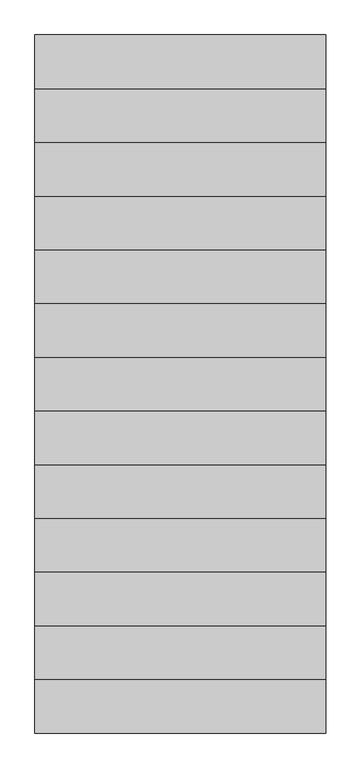
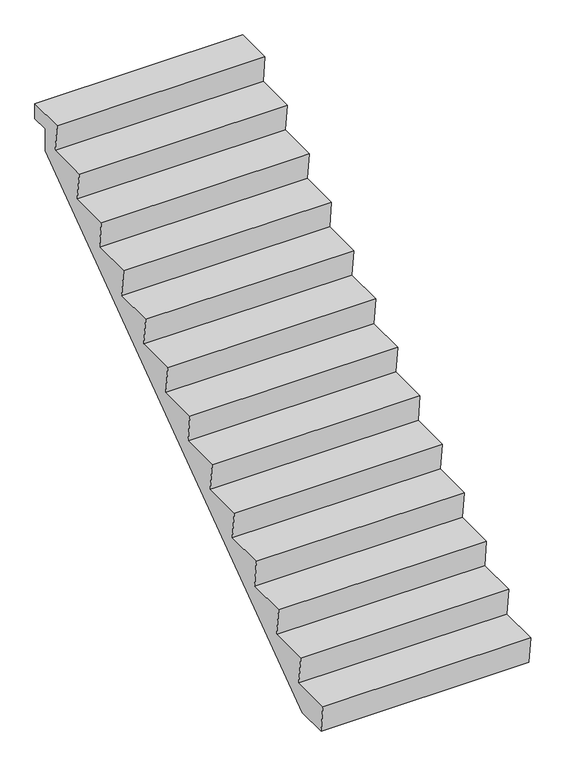
"""IFC4 building model written with IfcOpenShell, lengths in millimetres: stair geometry, NLRS_24_GM_LB_rechte steektrap prefab-AV_gen_rsf : prefab trap_gen__aant=12 b=1200 a=220 o=172.7 zonder bomen."""

from ifc_helpers import new_model, si_unit, frame, origin, place, context, project, spatial, polyline, outline, extrude, source, transform, mapped, element, save


def stair_322cbe82(model_context):
    return source(origin(), model_context, "Body", "SweptSolid", [
        extrude(outline(polyline([(2880.0, 2270.0), (3120.0, 2270.0), (3120.0, 2170.0), (3010.0, 2170.0), (3010.0, 2027.0164203), (223.9686206, 0.0), (20.0, 0.0), (0.0, 174.6153846), (260.0, 174.6153846), (240.0, 349.2307692), (500.0, 349.2307692), (480.0, 523.8461538), (740.0, 523.8461538), (720.0, 698.4615385), (980.0, 698.4615385), (960.0, 873.0769231), (1220.0, 873.0769231), (1200.0, 1047.6923077), (1460.0, 1047.6923077), (1440.0, 1222.3076923), (1700.0, 1222.3076923), (1680.0, 1396.9230769), (1940.0, 1396.9230769), (1920.0, 1571.5384615), (2180.0, 1571.5384615), (2160.0, 1746.1538462), (2420.0, 1746.1538462), (2400.0, 1920.7692308), (2660.0, 1920.7692308), (2640.0, 2095.3846154), (2900.0, 2095.3846154), (2880.0, 2270.0)])), frame((-650.0, 0.0, 0.0), z_axis=(1.0, 0.0, 0.0), x_axis=(0.0, 1.0, 0.0)), (0.0, 0.0, 1.0), 1300.0),
    ])


if __name__ == "__main__":
    model = new_model("IFC4")
    model_context = context("Model", 3, world=origin())
    ifc_project = project(units=[si_unit("LENGTHUNIT", "METRE", prefix="MILLI")], contexts=[model_context])
    site = spatial("IfcSite", under=ifc_project)
    building = spatial("IfcBuilding", under=site)
    placement = place(None, origin())
    stair_shape = stair_322cbe82(model_context)
    element("IfcStair", 1, ObjectType="NLRS_24_GM_LB_rechte steektrap prefab-AV_gen_rsf : prefab trap_gen__aant=12 b=1200 a=220 o=172.7 zonder bomen", at=placement, inside=building, context=model_context, shape_type="MappedRepresentation", body=[
        mapped(stair_shape, transform((0.0, 0.0, 0.0), x_axis=(1.0, 0.0, 0.0), y_axis=(0.0, 1.0, 0.0), z_axis=(0.0, 0.0, 1.0))),
    ])
    save(model, "model.ifc")

# Revit data of these elements
# Type "NLRS_24_GM_LB_rechte steektrap prefab-AV_gen_rsf : prefab trap_gen__aant=12 b=1200 a=220 o=172.7 zonder bomen"
#   IfcExportAs = "IfcStair"
#   Type Comments = " "
#   Model = " "
#   Manufacturer = " "
#   Keynote = " "
#   Description = "rechte steektrap prefab\r\naant=11 b=1200 a=220 o=181,8\r\nzonder bomen"
#   Assembly Code = "24.11"
#   Aantrede onder = 240 mm
#   Width = 1300 mm
#   Wel diepte = 20 mm
#   Trapboom breedte = 0 mm
#   Thickness = 120 mm
#   Optrede onderste trede = 150 mm
#   NLRS_C_lengte = 2880 mm
#   Length = 3360 mm
#   Hoogte oplegnok onder = 100 mm
#   Hoogte oplegnok boven = 100 mm
#   Height = 2270 mm
#   Breedte oplegnok boven = 110 mm
#   BottomCalc = 150 mm
#   Actual Tread Depth = 240 mm
#   Actual Riser Height = 174.615 mm
#   Actual Number of Tread = 12
#   Actual Number of Risers = 13
#   Aantrede boven = 240 mm
#   Aantal treden max dertig = 13
#   Trapboom = no
#   Oplegnok onder = no
#   NLRS_C_materiaal = NLRS_f2_beton prefab_gen_rsf
#   Default Elevation = 0
# Element 1 (IfcStair, "NLRS_24_GM_LB_rechte steektrap prefab-AV_gen_rsf : prefab trap_gen__aant=12 b=1200 a=220 o=172.7 zonder bomen")
#   Materials on its faces: "NLRS_f2_beton prefab_gen_rsf"
# Materials
#   "NLRS_f2_beton prefab_gen_rsf": class "F - Niet gebakken kunststeen", colour RGB 129 133 118, transparency 0, Keynote = "f2", Manufacturer = "Revit Standards Foundation", URL = "www.revitstandards.org", Description = "beton prefab", Cost = 0
